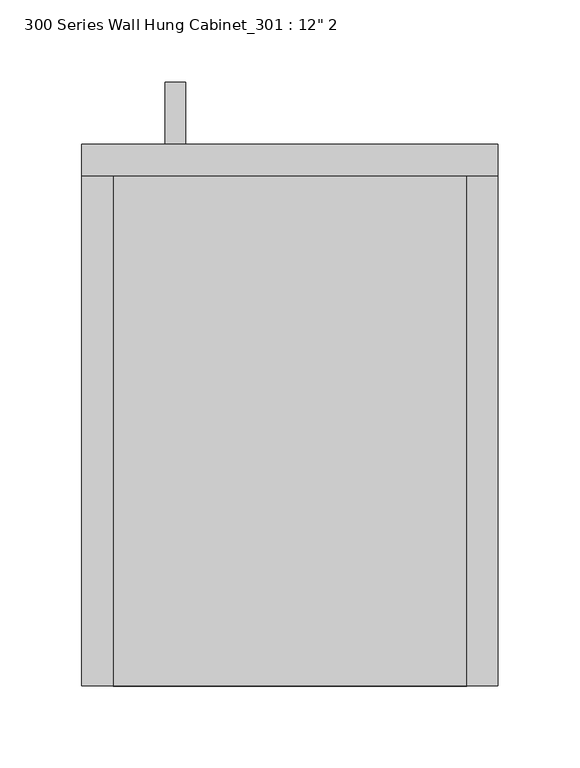
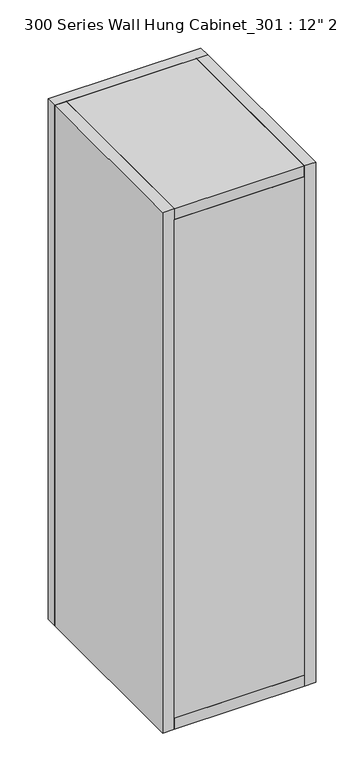
"""IFC4 building model written with IfcOpenShell, lengths in millimetres: furniture geometry."""

from ifc_helpers import new_model, si_unit, frame, origin, place, context, project, spatial, polyline, outline, extrude, source, transform, mapped, element, save


def furniture_3e0bc3ae(model_context):
    return source(origin(), model_context, "Body", "SweptSolid", [
        extrude(outline(polyline([(390.525, 1352.5425373), (390.525, 1365.2121874), (428.6060937, 1365.2121874), (428.6060937, 1270.0), (390.525, 1270.0), (390.525, 1282.6696501), (415.9364436, 1282.6696501), (415.9364436, 1352.5425373), (390.525, 1352.5425373)])), frame((-76.2, 0.0, 0.0), z_axis=(1.0, 0.0, 0.0), x_axis=(0.0, 1.0, 0.0)), (0.0, 0.0, 1.0), 12.4065288),
        extrude(outline(polyline([(107.95, 371.475), (107.95, 60.325), (-107.95, 60.325), (-107.95, 371.475), (107.95, 371.475)])), frame((0.0, 0.0, 1219.2), z_axis=(0.0, 0.0, 1.0), x_axis=(1.0, 0.0, 0.0)), (0.0, 0.0, 1.0), 19.05),
        extrude(outline(polyline([(107.95, 60.325), (-107.95, 60.325), (-107.95, 79.375), (107.95, 79.375), (107.95, 60.325)])), frame((0.0, 0.0, 1238.25), z_axis=(0.0, 0.0, 1.0), x_axis=(1.0, 0.0, 0.0)), (0.0, 0.0, 1.0), 876.3),
        extrude(outline(polyline([(127.0, 371.475), (-127.0, 371.475), (-127.0, 390.525), (127.0, 390.525), (127.0, 371.475)])), frame((0.0, 0.0, 1219.2), z_axis=(0.0, 0.0, 1.0), x_axis=(1.0, 0.0, 0.0)), (0.0, 0.0, 1.0), 914.4),
        extrude(outline(polyline([(-127.0, 60.325), (-127.0, 371.475), (-107.95, 371.475), (-107.95, 60.325), (-127.0, 60.325)])), frame((0.0, 0.0, 1219.2), z_axis=(0.0, 0.0, 1.0), x_axis=(1.0, 0.0, 0.0)), (0.0, 0.0, 1.0), 914.4),
        extrude(outline(polyline([(107.95, 60.325), (107.95, 371.475), (127.0, 371.475), (127.0, 60.325), (107.95, 60.325)])), frame((0.0, 0.0, 1219.2), z_axis=(0.0, 0.0, 1.0), x_axis=(1.0, 0.0, 0.0)), (0.0, 0.0, 1.0), 914.4),
        extrude(outline(polyline([(107.95, 371.475), (107.95, 60.325), (-107.95, 60.325), (-107.95, 371.475), (107.95, 371.475)])), frame((0.0, 0.0, 2114.55), z_axis=(0.0, 0.0, 1.0), x_axis=(1.0, 0.0, 0.0)), (0.0, 0.0, 1.0), 19.05),
    ])


if __name__ == "__main__":
    model = new_model("IFC4")
    model_context = context("Model", 3, world=origin())
    ifc_project = project(units=[si_unit("LENGTHUNIT", "METRE", prefix="MILLI")], contexts=[model_context])
    site = spatial("IfcSite", under=ifc_project)
    building = spatial("IfcBuilding", under=site)
    placement = place(None, origin())
    furniture_shape = furniture_3e0bc3ae(model_context)
    element("IfcFurniture", 1, ObjectType="300 Series Wall Hung Cabinet_301 : 12\" 2", at=placement, inside=building, context=model_context, shape_type="MappedRepresentation", body=[
        mapped(furniture_shape, transform((0.0, 0.0, 0.0), x_axis=(1.0, 0.0, 0.0), y_axis=(0.0, 1.0, 0.0), z_axis=(0.0, 0.0, 1.0))),
    ])
    save(model, "model.ifc")

# Revit data of these elements
# Type "300 Series Wall Hung Cabinet_301 : 12\" 2"
#   URL = "www.wicnet.org/manual_sections.asp"
#   Model = "301"
#   Manufacturer = "Woodwork Institute"
#   Description = "Wall Hung Cabinet"
#   Content Creator URL = "www.AECcontent.com"
#   Content Creator = "AECcontent"
#   Assembly Code = "E2010200"
#   Width = 0' - 10"
#   Top of Cabinet = 7' - 0"
#   Height = 3' - 0"
#   Depth = 1' - 1"
#   Top Panel Material = none
#   Side Panel Material = none
#   Door Panel Material = none
#   Shelf Panel Material = none
# Element 1 (IfcFurniture, "300 Series Wall Hung Cabinet_301 : 12\" 2")
#   Materials on its faces: "CASEWORK"
# Materials
#   "CASEWORK": class "Generic", colour RGB 181 181 181, transparency 0, Cost = 0
